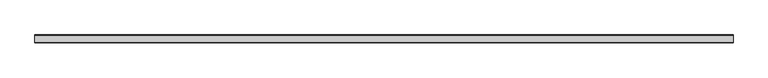
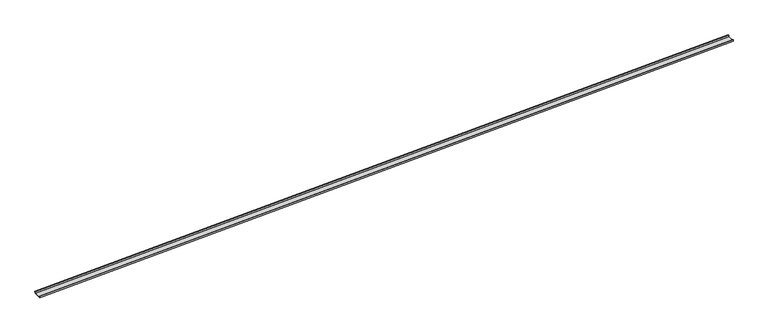
"""IFC4 building model written with IfcOpenShell, lengths in millimetres: proxy geometry, Generic Models 2:Generic Models 2:310765:Generic Models 2:310765 : Generic Models 2:Generic Models 2:310765:147 : Generic Models 2:Generic Models 2:310765:Generic Models 2:310765 : Generic Models 2:Generic Models 2:310765:300385."""

import ifcopenshell
import ifcopenshell.guid

model = None  # the IFC model being written
_history = None  # IfcOwnerHistory: only IFC2X3 demands one
_inside = {}  # id of a spatial element -> (the spatial element, [elements in it])
_under = {}  # id of a project, library or spatial element -> (it, [spatial elements below it])
_declared = {}  # id of a project -> (the project, [libraries it declares])
_typed = {}  # id of a type object -> (the type object, [elements of that type])
_made_of = {}  # id of a material, layer set ... -> (it, [elements and type objects made of it])


def new_model(schema):
    """Start an empty IFC model of exactly this schema.

    Asked for "IFC4X3", IfcOpenShell would pick the latest addendum, in which some entities
    have other attributes; the version numbers below select the first issue.
    IFC2X3 requires an IfcOwnerHistory on every rooted entity: one is made here for all.
    """
    global model, _history
    if schema == "IFC4X3":
        model = ifcopenshell.file(schema_version=(4, 3, 0, 0))
    else:
        model = ifcopenshell.file(schema=schema)
    _inside.clear()
    _under.clear()
    _declared.clear()
    _typed.clear()
    _made_of.clear()
    _history = None
    if model.schema == "IFC2X3":
        org = make("IfcOrganization", Name="unknown")
        user = make(
            "IfcPersonAndOrganization",
            ThePerson=make("IfcPerson", FamilyName="unknown"),
            TheOrganization=org,
        )
        app = make(
            "IfcApplication",
            ApplicationDeveloper=org,
            Version="unknown",
            ApplicationFullName="unknown",
            ApplicationIdentifier="unknown",
        )
        _history = make(
            "IfcOwnerHistory",
            OwningUser=user,
            OwningApplication=app,
            ChangeAction="ADDED",
            CreationDate=0,
        )
    return model


def make(cls, **values):
    """One entity of the class cls with the attributes given. An attribute that is None is left unset."""
    return model.create_entity(
        cls, **{name: value for name, value in values.items() if value is not None}
    )


def rooted(cls, **values):
    """An entity with a GlobalId (a new one), such as an element, a storey or a relation."""
    return make(cls, GlobalId=ifcopenshell.guid.new(), OwnerHistory=_history, **values)


def si_unit(unit_type, name, prefix=None):
    """IfcSIUnit, for example si_unit("LENGTHUNIT", "METRE", prefix="MILLI")."""
    return make("IfcSIUnit", UnitType=unit_type, Prefix=prefix, Name=name)


def assignment(units):
    """IfcUnitAssignment: the units of a project."""
    return None if units is None else make("IfcUnitAssignment", Units=units)


def point(xyz):
    """IfcCartesianPoint."""
    return None if xyz is None else make("IfcCartesianPoint", Coordinates=xyz)


def direction(xyz):
    """IfcDirection."""
    return None if xyz is None else make("IfcDirection", DirectionRatios=xyz)


def frame(location, z_axis=None, x_axis=None):
    """IfcAxis2Placement3D, a coordinate frame: its origin and axes. An axis left out is left unset."""
    return make(
        "IfcAxis2Placement3D",
        Location=point(location),
        Axis=direction(z_axis),
        RefDirection=direction(x_axis),
    )


def origin():
    """The frame at (0, 0, 0) with its axes left unset."""
    return frame((0.0, 0.0, 0.0))


def place(relative_to, where):
    """IfcLocalPlacement: puts the frame where relative to a parent placement (None: the world)."""
    return make(
        "IfcLocalPlacement", PlacementRelTo=relative_to, RelativePlacement=where
    )


def context(
    kind, dimensions, precision=None, world=None, true_north=None, identifier=None
):
    """IfcGeometricRepresentationContext, for example the 3D "Model" context."""
    return make(
        "IfcGeometricRepresentationContext",
        ContextIdentifier=identifier,
        ContextType=kind,
        CoordinateSpaceDimension=dimensions,
        Precision=precision,
        WorldCoordinateSystem=world,
        TrueNorth=true_north,
    )


def project(units=None, contexts=None):
    """IfcProject with its units and contexts."""
    return rooted(
        "IfcProject",
        Name="project",
        RepresentationContexts=contexts,
        UnitsInContext=assignment(units),
    )


def spatial(cls, under=None, at=None, **own):
    """A site, building, storey or space (cls), placed at a placement, below another one or the project."""
    s = rooted(cls, ObjectPlacement=at, **own)
    if under is not None:
        _under.setdefault(under.id(), (under, []))[1].append(s)
    return s


def polyline(points):
    """IfcPolyline through the points."""
    return make("IfcPolyline", Points=[point(p) for p in points])


def outline(outer, holes=None, kind="AREA"):
    """IfcArbitraryClosedProfileDef: a profile drawn as a closed curve; with holes, ...WithVoids."""
    if holes is None:
        return make("IfcArbitraryClosedProfileDef", ProfileType=kind, OuterCurve=outer)
    return make(
        "IfcArbitraryProfileDefWithVoids",
        ProfileType=kind,
        OuterCurve=outer,
        InnerCurves=holes,
    )


def extrude(swept, where, along, depth):
    """IfcExtrudedAreaSolid: the profile swept, set in the frame where, extruded along a direction by depth."""
    return make(
        "IfcExtrudedAreaSolid",
        SweptArea=swept,
        Position=where,
        ExtrudedDirection=direction(along),
        Depth=depth,
    )


def shape(context_of_items, identifier, shape_type, items):
    """IfcShapeRepresentation: the items that make up one representation, for example the "Body"."""
    return make(
        "IfcShapeRepresentation",
        ContextOfItems=context_of_items,
        RepresentationIdentifier=identifier,
        RepresentationType=shape_type,
        Items=items,
    )


def source(mapping_origin, context_of_items, identifier, shape_type, items):
    """IfcRepresentationMap: a shape defined once, which mapped items show again and again."""
    return make(
        "IfcRepresentationMap",
        MappingOrigin=mapping_origin,
        MappedRepresentation=shape(context_of_items, identifier, shape_type, items),
    )


def transform(
    local_origin,
    x_axis=None,
    y_axis=None,
    z_axis=None,
    scale=None,
    scale2=None,
    scale3=None,
    uniform=True,
):
    """IfcCartesianTransformationOperator3D, or its non-uniform kind. x_axis, y_axis, z_axis: its Axis1, 2, 3."""
    if uniform:
        return make(
            "IfcCartesianTransformationOperator3D",
            Axis1=direction(x_axis),
            Axis2=direction(y_axis),
            LocalOrigin=point(local_origin),
            Scale=scale,
            Axis3=direction(z_axis),
        )
    return make(
        "IfcCartesianTransformationOperator3DnonUniform",
        Axis1=direction(x_axis),
        Axis2=direction(y_axis),
        LocalOrigin=point(local_origin),
        Scale=scale,
        Axis3=direction(z_axis),
        Scale2=scale2,
        Scale3=scale3,
    )


def mapped(mapping_source, mapping_target):
    """IfcMappedItem: shows the shape of a source again, moved by a transform."""
    return make(
        "IfcMappedItem", MappingSource=mapping_source, MappingTarget=mapping_target
    )


def made_of(thing, what):
    """Note that an element or type object is made of a material, layer set ...; save() writes the relation."""
    if what is not None:
        _made_of.setdefault(what.id(), (what, []))[1].append(thing)
    return thing


def element(
    cls,
    number,
    at=None,
    inside=None,
    cuts=None,
    type_object=None,
    material=None,
    context=None,
    identifier="Body",
    shape_type=None,
    held_by="IfcProductDefinitionShape",
    body=None,
    shapes=None,
    **own,
):
    """One element of the class cls, such as IfcWall. Its Tag is "e" and its number.

    at: its placement. inside: the storey or other place that contains it. cuts: it is an
    opening in that element (IfcRelVoidsElement). A single representation is given by context,
    identifier, shape_type and body (its items); several are given by shapes. held_by: the class
    of the entity that holds the representations. save() writes the other relations.
    """
    e = rooted(cls, Tag="e%d" % number, ObjectPlacement=at, **own)
    if body is not None:
        shapes = [shape(context, identifier, shape_type, body)]
    if shapes is not None:
        e.Representation = make(held_by, Representations=shapes)
    if inside is not None:
        _inside.setdefault(inside.id(), (inside, []))[1].append(e)
    if cuts is not None:
        rooted(
            "IfcRelVoidsElement", RelatingBuildingElement=cuts, RelatedOpeningElement=e
        )
    if type_object is not None:
        _typed.setdefault(type_object.id(), (type_object, []))[1].append(e)
    return made_of(e, material)


def aggregate(whole, parts):
    """IfcRelAggregates: a whole, such as a stair, and the parts it consists of."""
    return rooted("IfcRelAggregates", RelatingObject=whole, RelatedObjects=parts)


def save(model, path):
    """Write the relations noted so far, then the file.

    IfcRelAggregates (storeys below a building ...), IfcRelContainedInSpatialStructure (elements
    in a storey), IfcRelDefinesByType, IfcRelAssociatesMaterial and IfcRelDeclares: one each for
    every whole, place, type object, material and project.
    """
    for whole, parts in _under.values():
        aggregate(whole, parts)
    for where, things in _inside.values():
        rooted(
            "IfcRelContainedInSpatialStructure",
            RelatedElements=things,
            RelatingStructure=where,
        )
    for kind, things in _typed.values():
        rooted("IfcRelDefinesByType", RelatedObjects=things, RelatingType=kind)
    for what, things in _made_of.values():
        rooted("IfcRelAssociatesMaterial", RelatedObjects=things, RelatingMaterial=what)
    for by, libraries in _declared.values():
        rooted("IfcRelDeclares", RelatingContext=by, RelatedDefinitions=libraries)
    model.write(path)


def generic_models_87d7309c(model_context):
    return source(origin(), model_context, "Body", "SweptSolid", [
        extrude(outline(polyline([(1.5875, 0.0), (1.5875, 50.8), (223.8375, 50.8), (223.8375, 1.5874999), (222.25, 1.5874999), (222.25, 49.2124999), (3.175, 49.2124999), (3.175, -1.5875), (-14.2875, -1.5875), (-14.2875, 9.525), (-12.7, 9.525), (-12.7, 0.0), (1.5875, 0.0)])), frame((558060.6329583, -578522.5893007, 3904.6995643), z_axis=(0.9991330730923568, 0.0, 0.041630544712067834), x_axis=(0.0, -1.0, 0.0)), (0.0, 0.0, 1.0), 21007.9629603),
    ])


if __name__ == "__main__":
    model = new_model("IFC4")
    model_context = context("Model", 3, world=origin())
    ifc_project = project(units=[si_unit("LENGTHUNIT", "METRE", prefix="MILLI")], contexts=[model_context])
    site = spatial("IfcSite", under=ifc_project)
    building = spatial("IfcBuilding", under=site)
    placement = place(None, origin())
    generic_models_shape = generic_models_87d7309c(model_context)
    element("IfcBuildingElementProxy", 1, Name="Generic Models 2:Generic Models 2:310765:Generic Models 2:310765 : Generic Models 2:Generic Models 2:310765:147 : Generic Models 2:Generic Models 2:310765:Generic Models 2:310765 : Generic Models 2:Generic Models 2:310765:300385", ObjectType="Generic Models 2:Generic Models 2:310765:Generic Models 2:310765 : Generic Models 2:Generic Models 2:310765:147 : Generic Models 2:Generic Models 2:310765:Generic Models 2:310765 : Generic Models 2:Generic Models 2:310765:300385", at=placement, inside=building, context=model_context, shape_type="MappedRepresentation", body=[
        mapped(generic_models_shape, transform((0.0, 0.0, 0.0), x_axis=(1.0, 0.0, 0.0), y_axis=(0.0, 1.0, 0.0), z_axis=(0.0, 0.0, 1.0))),
    ])
    save(model, "model.ifc")

# Revit data of these elements
# Type "Generic Models 2:Generic Models 2:310765:Generic Models 2:310765 : Generic Models 2:Generic Models 2:310765:147 : Generic Models 2:Generic Models 2:310765:Generic Models 2:310765 : Generic Models 2:Generic Models 2:310765:300385"
#   NameOverride = "Generic Models 2:Generic Models 2:310765:Generic Models 2:310765 : Generic Models 2:Generic Models 2:310765:300385"
#   ObjectTypeOverride = "Generic Models 2:310765 : Generic Models 2:Generic Models 2:310765"
#   Reference = "Generic Models 2"
#   Tag = "300385"
# Element 1 (IfcBuildingElementProxy, "Generic Models 2:Generic Models 2:310765:Generic Models 2:310765 : Generic Models 2:Generic Models 2:310765:147 : Generic Models 2:Generic Models 2:310765:Generic Models 2:310765 : Generic Models 2:Generic Models 2:310765:300385")
#   Materials on its faces: "STRUCTURAL STANDING SEAM SHEET METAL ROOFING - BATTENLOK - COLOR T.B.D."
# Materials
#   "STRUCTURAL STANDING SEAM SHEET METAL ROOFING - BATTENLOK - COLOR T.B.D.": class "Generic", colour RGB 120 120 120, transparency 0, Cost = 0
